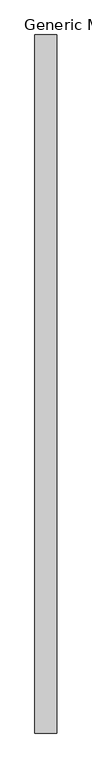
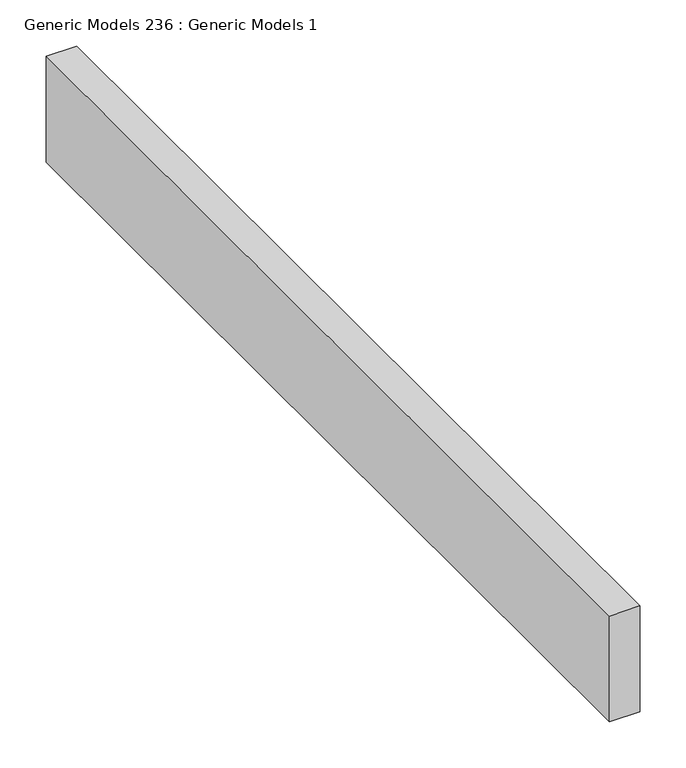
"""IFC4 building model written with IfcOpenShell, lengths in millimetres: proxy geometry, Generic Models 236 : Generic Models 1."""

import ifcopenshell
import ifcopenshell.guid

model = None  # the IFC model being written
_history = None  # IfcOwnerHistory: only IFC2X3 demands one
_inside = {}  # id of a spatial element -> (the spatial element, [elements in it])
_under = {}  # id of a project, library or spatial element -> (it, [spatial elements below it])
_declared = {}  # id of a project -> (the project, [libraries it declares])
_typed = {}  # id of a type object -> (the type object, [elements of that type])
_made_of = {}  # id of a material, layer set ... -> (it, [elements and type objects made of it])


def new_model(schema):
    """Start an empty IFC model of exactly this schema.

    Asked for "IFC4X3", IfcOpenShell would pick the latest addendum, in which some entities
    have other attributes; the version numbers below select the first issue.
    IFC2X3 requires an IfcOwnerHistory on every rooted entity: one is made here for all.
    """
    global model, _history
    if schema == "IFC4X3":
        model = ifcopenshell.file(schema_version=(4, 3, 0, 0))
    else:
        model = ifcopenshell.file(schema=schema)
    _inside.clear()
    _under.clear()
    _declared.clear()
    _typed.clear()
    _made_of.clear()
    _history = None
    if model.schema == "IFC2X3":
        org = make("IfcOrganization", Name="unknown")
        user = make(
            "IfcPersonAndOrganization",
            ThePerson=make("IfcPerson", FamilyName="unknown"),
            TheOrganization=org,
        )
        app = make(
            "IfcApplication",
            ApplicationDeveloper=org,
            Version="unknown",
            ApplicationFullName="unknown",
            ApplicationIdentifier="unknown",
        )
        _history = make(
            "IfcOwnerHistory",
            OwningUser=user,
            OwningApplication=app,
            ChangeAction="ADDED",
            CreationDate=0,
        )
    return model


def make(cls, **values):
    """One entity of the class cls with the attributes given. An attribute that is None is left unset."""
    return model.create_entity(
        cls, **{name: value for name, value in values.items() if value is not None}
    )


def rooted(cls, **values):
    """An entity with a GlobalId (a new one), such as an element, a storey or a relation."""
    return make(cls, GlobalId=ifcopenshell.guid.new(), OwnerHistory=_history, **values)


def si_unit(unit_type, name, prefix=None):
    """IfcSIUnit, for example si_unit("LENGTHUNIT", "METRE", prefix="MILLI")."""
    return make("IfcSIUnit", UnitType=unit_type, Prefix=prefix, Name=name)


def assignment(units):
    """IfcUnitAssignment: the units of a project."""
    return None if units is None else make("IfcUnitAssignment", Units=units)


def point(xyz):
    """IfcCartesianPoint."""
    return None if xyz is None else make("IfcCartesianPoint", Coordinates=xyz)


def direction(xyz):
    """IfcDirection."""
    return None if xyz is None else make("IfcDirection", DirectionRatios=xyz)


def frame(location, z_axis=None, x_axis=None):
    """IfcAxis2Placement3D, a coordinate frame: its origin and axes. An axis left out is left unset."""
    return make(
        "IfcAxis2Placement3D",
        Location=point(location),
        Axis=direction(z_axis),
        RefDirection=direction(x_axis),
    )


def origin():
    """The frame at (0, 0, 0) with its axes left unset."""
    return frame((0.0, 0.0, 0.0))


def place(relative_to, where):
    """IfcLocalPlacement: puts the frame where relative to a parent placement (None: the world)."""
    return make(
        "IfcLocalPlacement", PlacementRelTo=relative_to, RelativePlacement=where
    )


def context(
    kind, dimensions, precision=None, world=None, true_north=None, identifier=None
):
    """IfcGeometricRepresentationContext, for example the 3D "Model" context."""
    return make(
        "IfcGeometricRepresentationContext",
        ContextIdentifier=identifier,
        ContextType=kind,
        CoordinateSpaceDimension=dimensions,
        Precision=precision,
        WorldCoordinateSystem=world,
        TrueNorth=true_north,
    )


def project(units=None, contexts=None):
    """IfcProject with its units and contexts."""
    return rooted(
        "IfcProject",
        Name="project",
        RepresentationContexts=contexts,
        UnitsInContext=assignment(units),
    )


def spatial(cls, under=None, at=None, **own):
    """A site, building, storey or space (cls), placed at a placement, below another one or the project."""
    s = rooted(cls, ObjectPlacement=at, **own)
    if under is not None:
        _under.setdefault(under.id(), (under, []))[1].append(s)
    return s


def polyline(points):
    """IfcPolyline through the points."""
    return make("IfcPolyline", Points=[point(p) for p in points])


def outline(outer, holes=None, kind="AREA"):
    """IfcArbitraryClosedProfileDef: a profile drawn as a closed curve; with holes, ...WithVoids."""
    if holes is None:
        return make("IfcArbitraryClosedProfileDef", ProfileType=kind, OuterCurve=outer)
    return make(
        "IfcArbitraryProfileDefWithVoids",
        ProfileType=kind,
        OuterCurve=outer,
        InnerCurves=holes,
    )


def extrude(swept, where, along, depth):
    """IfcExtrudedAreaSolid: the profile swept, set in the frame where, extruded along a direction by depth."""
    return make(
        "IfcExtrudedAreaSolid",
        SweptArea=swept,
        Position=where,
        ExtrudedDirection=direction(along),
        Depth=depth,
    )


def shape(context_of_items, identifier, shape_type, items):
    """IfcShapeRepresentation: the items that make up one representation, for example the "Body"."""
    return make(
        "IfcShapeRepresentation",
        ContextOfItems=context_of_items,
        RepresentationIdentifier=identifier,
        RepresentationType=shape_type,
        Items=items,
    )


def source(mapping_origin, context_of_items, identifier, shape_type, items):
    """IfcRepresentationMap: a shape defined once, which mapped items show again and again."""
    return make(
        "IfcRepresentationMap",
        MappingOrigin=mapping_origin,
        MappedRepresentation=shape(context_of_items, identifier, shape_type, items),
    )


def transform(
    local_origin,
    x_axis=None,
    y_axis=None,
    z_axis=None,
    scale=None,
    scale2=None,
    scale3=None,
    uniform=True,
):
    """IfcCartesianTransformationOperator3D, or its non-uniform kind. x_axis, y_axis, z_axis: its Axis1, 2, 3."""
    if uniform:
        return make(
            "IfcCartesianTransformationOperator3D",
            Axis1=direction(x_axis),
            Axis2=direction(y_axis),
            LocalOrigin=point(local_origin),
            Scale=scale,
            Axis3=direction(z_axis),
        )
    return make(
        "IfcCartesianTransformationOperator3DnonUniform",
        Axis1=direction(x_axis),
        Axis2=direction(y_axis),
        LocalOrigin=point(local_origin),
        Scale=scale,
        Axis3=direction(z_axis),
        Scale2=scale2,
        Scale3=scale3,
    )


def mapped(mapping_source, mapping_target):
    """IfcMappedItem: shows the shape of a source again, moved by a transform."""
    return make(
        "IfcMappedItem", MappingSource=mapping_source, MappingTarget=mapping_target
    )


def made_of(thing, what):
    """Note that an element or type object is made of a material, layer set ...; save() writes the relation."""
    if what is not None:
        _made_of.setdefault(what.id(), (what, []))[1].append(thing)
    return thing


def element(
    cls,
    number,
    at=None,
    inside=None,
    cuts=None,
    type_object=None,
    material=None,
    context=None,
    identifier="Body",
    shape_type=None,
    held_by="IfcProductDefinitionShape",
    body=None,
    shapes=None,
    **own,
):
    """One element of the class cls, such as IfcWall. Its Tag is "e" and its number.

    at: its placement. inside: the storey or other place that contains it. cuts: it is an
    opening in that element (IfcRelVoidsElement). A single representation is given by context,
    identifier, shape_type and body (its items); several are given by shapes. held_by: the class
    of the entity that holds the representations. save() writes the other relations.
    """
    e = rooted(cls, Tag="e%d" % number, ObjectPlacement=at, **own)
    if body is not None:
        shapes = [shape(context, identifier, shape_type, body)]
    if shapes is not None:
        e.Representation = make(held_by, Representations=shapes)
    if inside is not None:
        _inside.setdefault(inside.id(), (inside, []))[1].append(e)
    if cuts is not None:
        rooted(
            "IfcRelVoidsElement", RelatingBuildingElement=cuts, RelatedOpeningElement=e
        )
    if type_object is not None:
        _typed.setdefault(type_object.id(), (type_object, []))[1].append(e)
    return made_of(e, material)


def aggregate(whole, parts):
    """IfcRelAggregates: a whole, such as a stair, and the parts it consists of."""
    return rooted("IfcRelAggregates", RelatingObject=whole, RelatedObjects=parts)


def save(model, path):
    """Write the relations noted so far, then the file.

    IfcRelAggregates (storeys below a building ...), IfcRelContainedInSpatialStructure (elements
    in a storey), IfcRelDefinesByType, IfcRelAssociatesMaterial and IfcRelDeclares: one each for
    every whole, place, type object, material and project.
    """
    for whole, parts in _under.values():
        aggregate(whole, parts)
    for where, things in _inside.values():
        rooted(
            "IfcRelContainedInSpatialStructure",
            RelatedElements=things,
            RelatingStructure=where,
        )
    for kind, things in _typed.values():
        rooted("IfcRelDefinesByType", RelatedObjects=things, RelatingType=kind)
    for what, things in _made_of.values():
        rooted("IfcRelAssociatesMaterial", RelatedObjects=things, RelatingMaterial=what)
    for by, libraries in _declared.values():
        rooted("IfcRelDeclares", RelatingContext=by, RelatedDefinitions=libraries)
    model.write(path)


def generic_models_236_generic_models_1_f8917e71(model_context):
    return source(origin(), model_context, "Body", "SweptSolid", [
        extrude(outline(polyline([(48507.65, 0.0), (48469.55, 0.0), (48469.55, 1219.2), (48507.65, 1219.2), (48507.65, 0.0)])), frame((0.0, 0.0, 5507.83125), z_axis=(0.0, 0.0, 1.0), x_axis=(1.0, 0.0, 0.0)), (0.0, 0.0, 1.0), 139.7),
    ])


if __name__ == "__main__":
    model = new_model("IFC4")
    model_context = context("Model", 3, world=origin())
    ifc_project = project(units=[si_unit("LENGTHUNIT", "METRE", prefix="MILLI")], contexts=[model_context])
    site = spatial("IfcSite", under=ifc_project)
    building = spatial("IfcBuilding", under=site)
    placement = place(None, origin())
    generic_models_236_generic_models_1_shape = generic_models_236_generic_models_1_f8917e71(model_context)
    element("IfcBuildingElementProxy", 1, Name="Generic Models 236 : Generic Models 1", ObjectType="Generic Models 236 : Generic Models 1", at=placement, inside=building, context=model_context, shape_type="MappedRepresentation", body=[
        mapped(generic_models_236_generic_models_1_shape, transform((0.0, 0.0, 0.0), x_axis=(1.0, 0.0, 0.0), y_axis=(0.0, 1.0, 0.0), z_axis=(0.0, 0.0, 1.0))),
    ])
    save(model, "model.ifc")

# Revit data of these elements
# Element 1 (IfcBuildingElementProxy, "Generic Models 236 : Generic Models 1")
#   Materials on its faces: "EXISTING RIM BOARD OR JOIST"
# Materials
#   "EXISTING RIM BOARD OR JOIST": class "Wood", colour RGB 234 198 147, transparency 0, Description = "Pinus Echinata", Cost = 0
